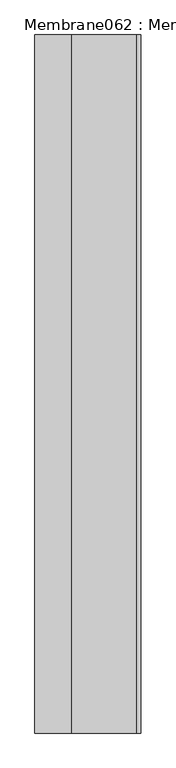
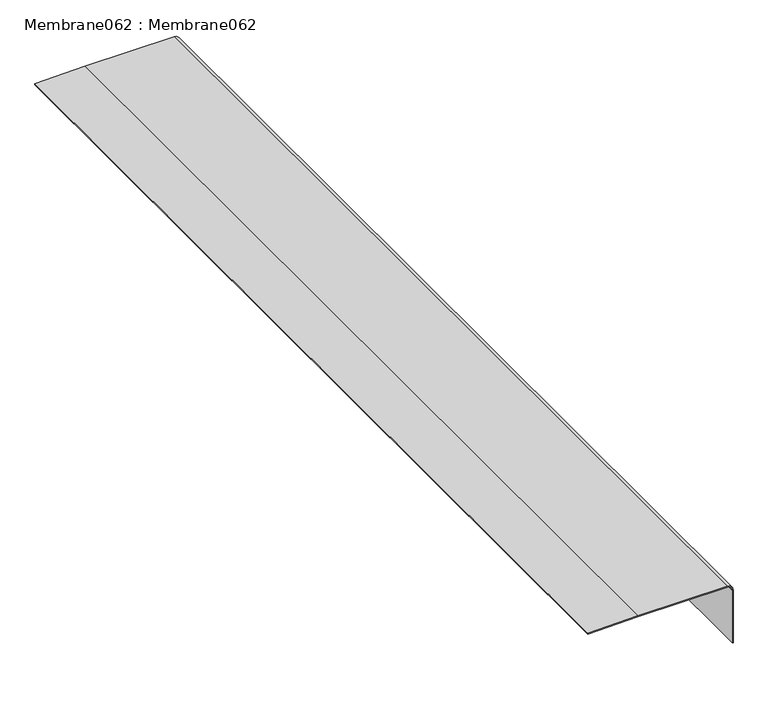
"""IFC4 building model written with IfcOpenShell, lengths in millimetres: proxy geometry, Membrane062 : Membrane062."""

import ifcopenshell
import ifcopenshell.guid

model = None  # the IFC model being written
_history = None  # IfcOwnerHistory: only IFC2X3 demands one
_inside = {}  # id of a spatial element -> (the spatial element, [elements in it])
_under = {}  # id of a project, library or spatial element -> (it, [spatial elements below it])
_declared = {}  # id of a project -> (the project, [libraries it declares])
_typed = {}  # id of a type object -> (the type object, [elements of that type])
_made_of = {}  # id of a material, layer set ... -> (it, [elements and type objects made of it])


def new_model(schema):
    """Start an empty IFC model of exactly this schema.

    Asked for "IFC4X3", IfcOpenShell would pick the latest addendum, in which some entities
    have other attributes; the version numbers below select the first issue.
    IFC2X3 requires an IfcOwnerHistory on every rooted entity: one is made here for all.
    """
    global model, _history
    if schema == "IFC4X3":
        model = ifcopenshell.file(schema_version=(4, 3, 0, 0))
    else:
        model = ifcopenshell.file(schema=schema)
    _inside.clear()
    _under.clear()
    _declared.clear()
    _typed.clear()
    _made_of.clear()
    _history = None
    if model.schema == "IFC2X3":
        org = make("IfcOrganization", Name="unknown")
        user = make(
            "IfcPersonAndOrganization",
            ThePerson=make("IfcPerson", FamilyName="unknown"),
            TheOrganization=org,
        )
        app = make(
            "IfcApplication",
            ApplicationDeveloper=org,
            Version="unknown",
            ApplicationFullName="unknown",
            ApplicationIdentifier="unknown",
        )
        _history = make(
            "IfcOwnerHistory",
            OwningUser=user,
            OwningApplication=app,
            ChangeAction="ADDED",
            CreationDate=0,
        )
    return model


def make(cls, **values):
    """One entity of the class cls with the attributes given. An attribute that is None is left unset."""
    return model.create_entity(
        cls, **{name: value for name, value in values.items() if value is not None}
    )


def rooted(cls, **values):
    """An entity with a GlobalId (a new one), such as an element, a storey or a relation."""
    return make(cls, GlobalId=ifcopenshell.guid.new(), OwnerHistory=_history, **values)


def si_unit(unit_type, name, prefix=None):
    """IfcSIUnit, for example si_unit("LENGTHUNIT", "METRE", prefix="MILLI")."""
    return make("IfcSIUnit", UnitType=unit_type, Prefix=prefix, Name=name)


def assignment(units):
    """IfcUnitAssignment: the units of a project."""
    return None if units is None else make("IfcUnitAssignment", Units=units)


def point(xyz):
    """IfcCartesianPoint."""
    return None if xyz is None else make("IfcCartesianPoint", Coordinates=xyz)


def direction(xyz):
    """IfcDirection."""
    return None if xyz is None else make("IfcDirection", DirectionRatios=xyz)


def frame(location, z_axis=None, x_axis=None):
    """IfcAxis2Placement3D, a coordinate frame: its origin and axes. An axis left out is left unset."""
    return make(
        "IfcAxis2Placement3D",
        Location=point(location),
        Axis=direction(z_axis),
        RefDirection=direction(x_axis),
    )


def frame_2d(location, x_axis=None):
    """IfcAxis2Placement2D, a coordinate frame in the plane: its origin and x axis."""
    return make(
        "IfcAxis2Placement2D", Location=point(location), RefDirection=direction(x_axis)
    )


def origin():
    """The frame at (0, 0, 0) with its axes left unset."""
    return frame((0.0, 0.0, 0.0))


def place(relative_to, where):
    """IfcLocalPlacement: puts the frame where relative to a parent placement (None: the world)."""
    return make(
        "IfcLocalPlacement", PlacementRelTo=relative_to, RelativePlacement=where
    )


def context(
    kind, dimensions, precision=None, world=None, true_north=None, identifier=None
):
    """IfcGeometricRepresentationContext, for example the 3D "Model" context."""
    return make(
        "IfcGeometricRepresentationContext",
        ContextIdentifier=identifier,
        ContextType=kind,
        CoordinateSpaceDimension=dimensions,
        Precision=precision,
        WorldCoordinateSystem=world,
        TrueNorth=true_north,
    )


def project(units=None, contexts=None):
    """IfcProject with its units and contexts."""
    return rooted(
        "IfcProject",
        Name="project",
        RepresentationContexts=contexts,
        UnitsInContext=assignment(units),
    )


def spatial(cls, under=None, at=None, **own):
    """A site, building, storey or space (cls), placed at a placement, below another one or the project."""
    s = rooted(cls, ObjectPlacement=at, **own)
    if under is not None:
        _under.setdefault(under.id(), (under, []))[1].append(s)
    return s


def polyline(points):
    """IfcPolyline through the points."""
    return make("IfcPolyline", Points=[point(p) for p in points])


def circle_curve(where, radius):
    """IfcCircle in the frame where."""
    return make("IfcCircle", Position=where, Radius=radius)


def trimmed(basis, trim1, trim2, sense, master):
    """IfcTrimmedCurve: the piece of a basis curve between two trims."""
    return make(
        "IfcTrimmedCurve",
        BasisCurve=basis,
        Trim1=trim1,
        Trim2=trim2,
        SenseAgreement=sense,
        MasterRepresentation=master,
    )


def segment(curve, same_sense, transition):
    """IfcCompositeCurveSegment."""
    return make(
        "IfcCompositeCurveSegment",
        Transition=transition,
        SameSense=same_sense,
        ParentCurve=curve,
    )


def composite_curve(segments, self_intersect=None):
    """IfcCompositeCurve: segments joined end to end."""
    return make("IfcCompositeCurve", Segments=segments, SelfIntersect=self_intersect)


def outline(outer, holes=None, kind="AREA"):
    """IfcArbitraryClosedProfileDef: a profile drawn as a closed curve; with holes, ...WithVoids."""
    if holes is None:
        return make("IfcArbitraryClosedProfileDef", ProfileType=kind, OuterCurve=outer)
    return make(
        "IfcArbitraryProfileDefWithVoids",
        ProfileType=kind,
        OuterCurve=outer,
        InnerCurves=holes,
    )


def extrude(swept, where, along, depth):
    """IfcExtrudedAreaSolid: the profile swept, set in the frame where, extruded along a direction by depth."""
    return make(
        "IfcExtrudedAreaSolid",
        SweptArea=swept,
        Position=where,
        ExtrudedDirection=direction(along),
        Depth=depth,
    )


def shape(context_of_items, identifier, shape_type, items):
    """IfcShapeRepresentation: the items that make up one representation, for example the "Body"."""
    return make(
        "IfcShapeRepresentation",
        ContextOfItems=context_of_items,
        RepresentationIdentifier=identifier,
        RepresentationType=shape_type,
        Items=items,
    )


def source(mapping_origin, context_of_items, identifier, shape_type, items):
    """IfcRepresentationMap: a shape defined once, which mapped items show again and again."""
    return make(
        "IfcRepresentationMap",
        MappingOrigin=mapping_origin,
        MappedRepresentation=shape(context_of_items, identifier, shape_type, items),
    )


def transform(
    local_origin,
    x_axis=None,
    y_axis=None,
    z_axis=None,
    scale=None,
    scale2=None,
    scale3=None,
    uniform=True,
):
    """IfcCartesianTransformationOperator3D, or its non-uniform kind. x_axis, y_axis, z_axis: its Axis1, 2, 3."""
    if uniform:
        return make(
            "IfcCartesianTransformationOperator3D",
            Axis1=direction(x_axis),
            Axis2=direction(y_axis),
            LocalOrigin=point(local_origin),
            Scale=scale,
            Axis3=direction(z_axis),
        )
    return make(
        "IfcCartesianTransformationOperator3DnonUniform",
        Axis1=direction(x_axis),
        Axis2=direction(y_axis),
        LocalOrigin=point(local_origin),
        Scale=scale,
        Axis3=direction(z_axis),
        Scale2=scale2,
        Scale3=scale3,
    )


def mapped(mapping_source, mapping_target):
    """IfcMappedItem: shows the shape of a source again, moved by a transform."""
    return make(
        "IfcMappedItem", MappingSource=mapping_source, MappingTarget=mapping_target
    )


def made_of(thing, what):
    """Note that an element or type object is made of a material, layer set ...; save() writes the relation."""
    if what is not None:
        _made_of.setdefault(what.id(), (what, []))[1].append(thing)
    return thing


def element(
    cls,
    number,
    at=None,
    inside=None,
    cuts=None,
    type_object=None,
    material=None,
    context=None,
    identifier="Body",
    shape_type=None,
    held_by="IfcProductDefinitionShape",
    body=None,
    shapes=None,
    **own,
):
    """One element of the class cls, such as IfcWall. Its Tag is "e" and its number.

    at: its placement. inside: the storey or other place that contains it. cuts: it is an
    opening in that element (IfcRelVoidsElement). A single representation is given by context,
    identifier, shape_type and body (its items); several are given by shapes. held_by: the class
    of the entity that holds the representations. save() writes the other relations.
    """
    e = rooted(cls, Tag="e%d" % number, ObjectPlacement=at, **own)
    if body is not None:
        shapes = [shape(context, identifier, shape_type, body)]
    if shapes is not None:
        e.Representation = make(held_by, Representations=shapes)
    if inside is not None:
        _inside.setdefault(inside.id(), (inside, []))[1].append(e)
    if cuts is not None:
        rooted(
            "IfcRelVoidsElement", RelatingBuildingElement=cuts, RelatedOpeningElement=e
        )
    if type_object is not None:
        _typed.setdefault(type_object.id(), (type_object, []))[1].append(e)
    return made_of(e, material)


def aggregate(whole, parts):
    """IfcRelAggregates: a whole, such as a stair, and the parts it consists of."""
    return rooted("IfcRelAggregates", RelatingObject=whole, RelatedObjects=parts)


def save(model, path):
    """Write the relations noted so far, then the file.

    IfcRelAggregates (storeys below a building ...), IfcRelContainedInSpatialStructure (elements
    in a storey), IfcRelDefinesByType, IfcRelAssociatesMaterial and IfcRelDeclares: one each for
    every whole, place, type object, material and project.
    """
    for whole, parts in _under.values():
        aggregate(whole, parts)
    for where, things in _inside.values():
        rooted(
            "IfcRelContainedInSpatialStructure",
            RelatedElements=things,
            RelatingStructure=where,
        )
    for kind, things in _typed.values():
        rooted("IfcRelDefinesByType", RelatedObjects=things, RelatingType=kind)
    for what, things in _made_of.values():
        rooted("IfcRelAssociatesMaterial", RelatedObjects=things, RelatingMaterial=what)
    for by, libraries in _declared.values():
        rooted("IfcRelDeclares", RelatingContext=by, RelatedDefinitions=libraries)
    model.write(path)


def membrane062_membrane062_aeca22a5(model_context):
    return source(origin(), model_context, "Body", "SweptSolid", [
        extrude(outline(composite_curve([segment(polyline([(40233.3001163, -4398.8442291), (40116.5801181, -4398.8442291), (40116.5801181, -4396.8442291), (40233.3001163, -4396.8442291)]), True, "CONTINUOUS"), segment(trimmed(circle_curve(frame_2d((40233.3001163, -4408.8442291)), 12.0), [point((40233.3001163, -4396.8442291))], [point((40245.3001163, -4408.8442291))], False, "CARTESIAN"), True, "CONTINUOUS"), segment(polyline([(40245.3001163, -4408.8442291), (40245.3001163, -4595.4560976), (40243.79743, -4699.8063764), (40241.7972226, -4699.8063764), (40243.3001163, -4595.4416982), (40243.3001163, -4408.8442291)]), True, "CONTINUOUS"), segment(trimmed(circle_curve(frame_2d((40233.3001163, -4408.8442291)), 10.0), [point((40243.3001163, -4408.8442291))], [point((40233.3001163, -4398.8442291))], True, "CARTESIAN"), True, "CONTINUOUS")], self_intersect=False)), frame((0.0, -1052.8906574, 0.0), z_axis=(0.0, 1.0, 0.0), x_axis=(0.0, 0.0, 1.0)), (0.0, 0.0, 1.0), 2000.0),
    ])


if __name__ == "__main__":
    model = new_model("IFC4")
    model_context = context("Model", 3, world=origin())
    ifc_project = project(units=[si_unit("LENGTHUNIT", "METRE", prefix="MILLI")], contexts=[model_context])
    site = spatial("IfcSite", under=ifc_project)
    building = spatial("IfcBuilding", under=site)
    placement = place(None, origin())
    membrane062_membrane062_shape = membrane062_membrane062_aeca22a5(model_context)
    element("IfcBuildingElementProxy", 1, Name="Membrane062 : Membrane062", ObjectType="Membrane062 : Membrane062", at=placement, inside=building, context=model_context, shape_type="MappedRepresentation", body=[
        mapped(membrane062_membrane062_shape, transform((0.0, 0.0, 0.0), x_axis=(1.0, 0.0, 0.0), y_axis=(0.0, 1.0, 0.0), z_axis=(0.0, 0.0, 1.0))),
    ])
    save(model, "model.ifc")

# Revit data of these elements
# Type "Membrane062 : Membrane062"
#   NameOverride = "Membrane062"
# Element 1 (IfcBuildingElementProxy, "Membrane062 : Membrane062")
#   Materials on its faces: "THREE PLY BUILT UP ROOF MEMBRANE"
# Materials
#   "THREE PLY BUILT UP ROOF MEMBRANE": class "Unassigned", colour RGB 63 63 63, transparency 0
